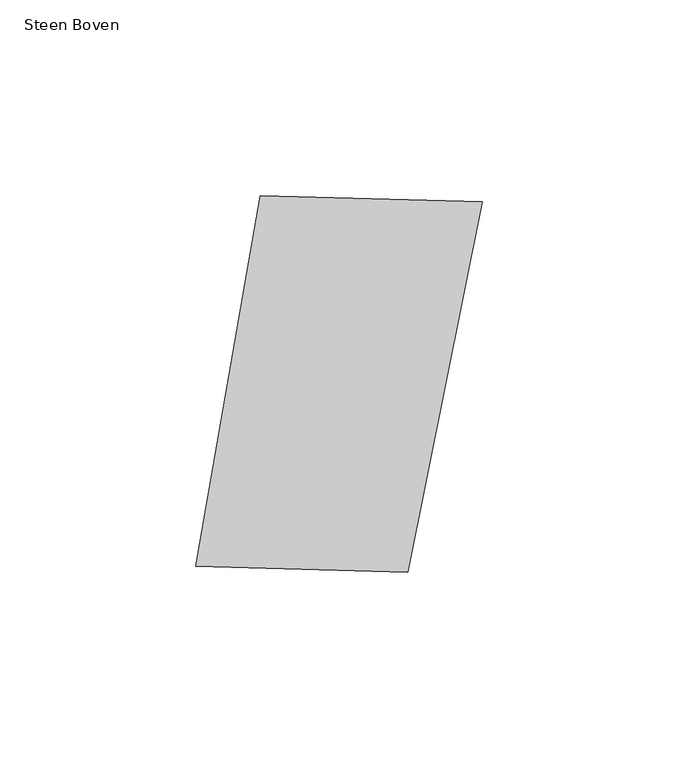
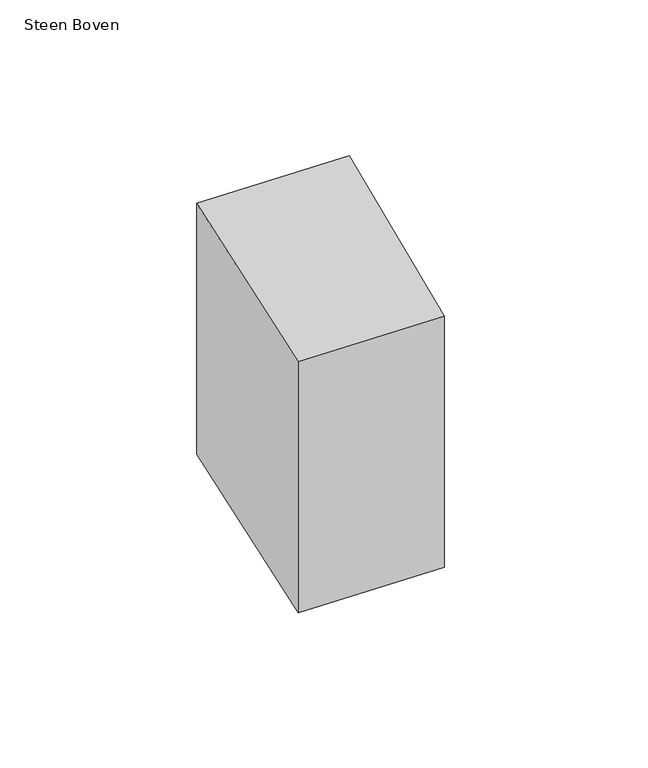
"""IFC4 building model written with IfcOpenShell, lengths in millimetres: proxy geometry, 00_GMA_steen_versie_4 : Steen Boven."""

from ifc_helpers import new_model, si_unit, origin, origin_with_axes, place, context, project, spatial, polyline, outline, extrude, source, transform, mapped, element, save


def steen_boven_e833c646(model_context):
    return source(origin(), model_context, "Body", "SweptSolid", [
        extrude(outline(polyline([(110.5378443, 118.4821388), (91.5555711, 23.8782157), (37.4465119, 25.323799), (53.890908, 119.9773726), (110.5378443, 118.4821388)])), origin_with_axes(), (0.0, 0.0, 1.0), 100.0),
    ])


if __name__ == "__main__":
    model = new_model("IFC4")
    model_context = context("Model", 3, world=origin())
    ifc_project = project(units=[si_unit("LENGTHUNIT", "METRE", prefix="MILLI")], contexts=[model_context])
    site = spatial("IfcSite", under=ifc_project)
    building = spatial("IfcBuilding", under=site)
    placement = place(None, origin())
    steen_boven_shape = steen_boven_e833c646(model_context)
    element("IfcBuildingElementProxy", 1, Name="00_GMA_steen_versie_4 : Steen Boven", ObjectType="00_GMA_steen_versie_4 : Steen Boven", at=placement, inside=building, context=model_context, shape_type="MappedRepresentation", body=[
        mapped(steen_boven_shape, transform((0.0, 0.0, 0.0), x_axis=(1.0, 0.0, 0.0), y_axis=(0.0, 1.0, 0.0), z_axis=(0.0, 0.0, 1.0))),
    ])
    save(model, "model.ifc")

# Revit data of these elements
# Type "00_GMA_steen_versie_4 : Steen Boven"
#   StootVoegHalfBoven [instance default] = 5 mm
#   StootVoegHalf [instance default] = 5 mm
#   StootVoegBreedteOnder = 10 mm
#   StootVoegBreedteBoven = 10 mm
#   Steendikte = 100 mm
#   LintVoegOnderHalf = 5 mm
#   LintVoegOnder = 10 mm
#   LintVoegBovenHalf = 0 mm
#   LintVoegBoven = 0 mm
#   materiaal = none
#   MateriaalVoeg = none
#   Default Elevation = 0
